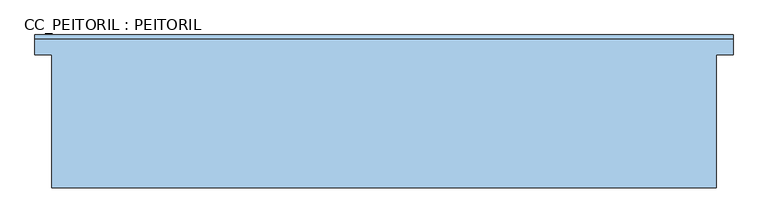
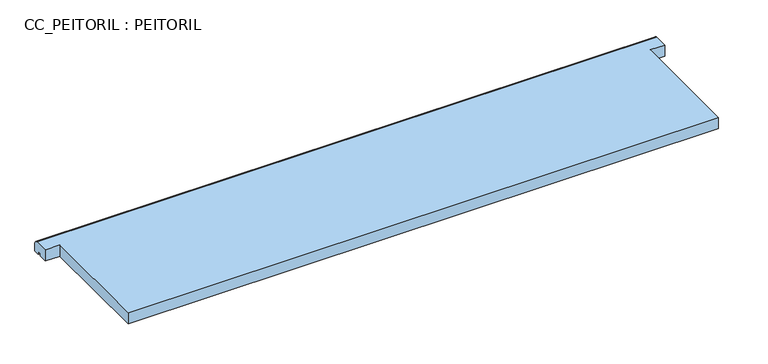
"""IFC4 building model written with IfcOpenShell, lengths in millimetres: window geometry, CC_PEITORIL : PEITORIL."""

from ifc_helpers import new_model, si_unit, frame, origin, place, context, project, spatial, circle_curve, source, transform, mapped, element, save
from ifc_brep_helpers import plane_surface, cylinder_surface, advanced_brep


def cc_peitoril_peitoril_2f67790e(model_context):
    return source(origin(), model_context, "Body", "AdvancedBrep", [
        advanced_brep(
        [(-500.0, 100.0, 1500.0), (-500.0, -100.0, 1500.0), (500.0, -100.0, 1500.0), (500.0, 100.0, 1500.0), (525.0, 100.0, 1500.0), (525.0, 123.4916648, 1500.0), (-525.0, 123.4916648, 1500.0), (-525.0, 100.0, 1500.0), (-500.0, 100.0, 1480.0), (-525.0, 100.0, 1480.0), (-525.0, 115.0, 1480.0), (525.0, 115.0, 1480.0), (525.0, 100.0, 1480.0), (500.0, 100.0, 1480.0), (500.0, -100.0, 1480.0), (-500.0, -100.0, 1480.0), (-525.0, 130.0, 1480.0), (525.0, 130.0, 1480.0), (525.0, 120.0, 1480.0), (-525.0, 120.0, 1480.0), (525.0, 115.0, 1485.0), (525.0, 120.0, 1485.0), (525.0, 130.0, 1493.4916648), (-525.0, 130.0, 1493.4916648), (-525.0, 120.0, 1485.0), (-525.0, 115.0, 1485.0)],
        [
            (0, 1),
            (1, 2),
            (2, 3),
            (3, 4),
            (4, 5),
            (5, 6),
            (6, 7),
            (7, 0),
            (8, 9),
            (9, 10),
            (10, 11),
            (11, 12),
            (12, 13),
            (13, 14),
            (14, 15),
            (15, 8),
            (16, 17),
            (17, 18),
            (18, 19),
            (19, 16),
            (0, 8),
            (15, 1),
            (14, 2),
            (13, 3),
            (12, 4),
            (11, 20),
            (20, 21),
            (21, 18),
            (17, 22),
            (22, 5, circle_curve(frame((525.0, 123.4916648, 1493.4916648), z_axis=(1.0, 0.0, 0.0), x_axis=(0.0, -1.0, 0.0)), 6.5083352)),
            (16, 23),
            (23, 22),
            (9, 7),
            (6, 23, circle_curve(frame((-525.0, 123.4916648, 1493.4916648), z_axis=(-1.0, 0.0, 0.0), x_axis=(0.0, -1.0, 0.0)), 6.5083352)),
            (19, 24),
            (24, 25),
            (25, 10),
            (24, 21),
            (20, 25),
        ],
        [
            plane_surface(frame((-500.0, -100.0, 1500.0), z_axis=(0.0, 0.0, 1.0), x_axis=(0.0, -1.0, 0.0))),
            plane_surface(frame((-500.0, -100.0, 1480.0), z_axis=(0.0, 0.0, -1.0), x_axis=(0.0, 1.0, 0.0))),
            plane_surface(frame((-500.0, 100.0, 1500.0), z_axis=(-1.0, 0.0, 0.0), x_axis=(0.0, 0.0, -1.0))),
            plane_surface(frame((-500.0, -100.0, 1500.0), z_axis=(0.0, -1.0, 0.0), x_axis=(0.0, 0.0, -1.0))),
            plane_surface(frame((500.0, -100.0, 1500.0), z_axis=(1.0, 0.0, 0.0), x_axis=(0.0, 0.0, -1.0))),
            plane_surface(frame((500.0, 100.0, 1500.0), z_axis=(0.0, -1.0, 0.0), x_axis=(0.0, 0.0, -1.0))),
            plane_surface(frame((525.0, 100.0, 1500.0), z_axis=(1.0, 0.0, 0.0), x_axis=(0.0, 0.0, -1.0))),
            plane_surface(frame((525.0, 130.0, 1500.0), z_axis=(0.0, 1.0, 0.0), x_axis=(0.0, 0.0, -1.0))),
            plane_surface(frame((-525.0, 130.0, 1500.0), z_axis=(-1.0, 0.0, 0.0), x_axis=(0.0, 0.0, -1.0))),
            plane_surface(frame((-525.0, 100.0, 1500.0), z_axis=(0.0, -1.0, 0.0), x_axis=(0.0, 0.0, -1.0))),
            cylinder_surface(frame((525.0, 123.4916648, 1493.4916648), z_axis=(-1.0, 0.0, 0.0), x_axis=(0.0, -1.0, 0.0)), 6.5083352),
            plane_surface(frame((-525.0, 115.0, 1485.0), z_axis=(0.0, 0.0, -1.0), x_axis=(1.0, 0.0, 0.0))),
            plane_surface(frame((-525.0, 120.0, 1485.0), z_axis=(0.0, -1.0, 0.0), x_axis=(1.0, 0.0, 0.0))),
            plane_surface(frame((-525.0, 115.0, 1480.0), z_axis=(0.0, 1.0, 0.0), x_axis=(1.0, 0.0, 0.0))),
        ],
        [
            (0, [[1, 2, 3, 4, 5, 6, 7, 8]]),
            (1, [[9, 10, 11, 12, 13, 14, 15, 16]]),
            (1, [[17, 18, 19, 20]]),
            (2, [[-1, 21, -16, 22]]),
            (3, [[-2, -22, -15, 23]]),
            (4, [[-3, -23, -14, 24]]),
            (5, [[-4, -24, -13, 25]]),
            (6, [[-25, -12, 26, 27, 28, -18, 29, 30, -5]]),
            (7, [[-17, 31, 32, -29]]),
            (8, [[33, -7, 34, -31, -20, 35, 36, 37, -10]]),
            (9, [[-8, -33, -9, -21]]),
            (10, [[-6, -30, -32, -34]]),
            (11, [[38, -27, 39, -36]]),
            (12, [[-38, -35, -19, -28]]),
            (13, [[-39, -26, -11, -37]]),
        ],
    ),
    ])


if __name__ == "__main__":
    model = new_model("IFC4")
    model_context = context("Model", 3, world=origin())
    ifc_project = project(units=[si_unit("LENGTHUNIT", "METRE", prefix="MILLI")], contexts=[model_context])
    site = spatial("IfcSite", under=ifc_project)
    building = spatial("IfcBuilding", under=site)
    placement = place(None, origin())
    cc_peitoril_peitoril_shape = cc_peitoril_peitoril_2f67790e(model_context)
    element("IfcWindow", 1, ObjectType="CC_PEITORIL : PEITORIL", at=placement, inside=building, context=model_context, shape_type="MappedRepresentation", body=[
        mapped(cc_peitoril_peitoril_shape, transform((0.0, 0.0, 0.0), x_axis=(1.0, 0.0, 0.0), y_axis=(0.0, 1.0, 0.0), z_axis=(0.0, 0.0, 1.0))),
    ])
    save(model, "model.ifc")

# Revit data of these elements
# Type "CC_PEITORIL : PEITORIL"
#   Type Mark = "PEITORIL"
#   Analytic Construction = "<Nenhum>"
#   Largura da pedra [instance default] = 0.26 m
#   Interna [instance default] = 0.08 m
#   Externa [instance default] = 0.008142 m
#   Extensão Exterior [instance default] = 0.03 m
#   Extensão Exterior Esquerda [instance default] = 0.085058 m
#   Extensão Exterior Direita [instance default] = 0.10 m
#   Espessura [instance default] = 0.02 m
#   Comprimento [instance default] = 1.00 m
#   Altura-padrão do peitoril = 1.48 m
#   ----EXTENSÃO---- [instance default] = 0.00 m
#   ----DEMAIS---- [instance default] = 0.00 m
#   Peitoril [instance default] = none
#   Rough Width = 0
#   Rough Height = 0
#   Height = 0
#   Wall Closure = (empty or 0)
#   Width = 0
# Element 1 (IfcWindow, "CC_PEITORIL : PEITORIL")
#   Interna = 0.00 m
#   Externa = 0.00 m
#   Extensão Exterior Esquerda = 0.025 m
#   Extensão Exterior Direita = 0.025 m
#   Peitoril = .GRANITO BRANCO ITAÚNAS
#   Materials on its faces: ".GRANITO BRANCO ITAÚNAS"
# Materials
#   ".GRANITO BRANCO ITAÚNAS": class ".CC_PEDRA REVEST.", colour RGB 202 195 174, transparency 0, Description = "Granito branco Itaúnas", Uso = "Pedra", Cost = 0
